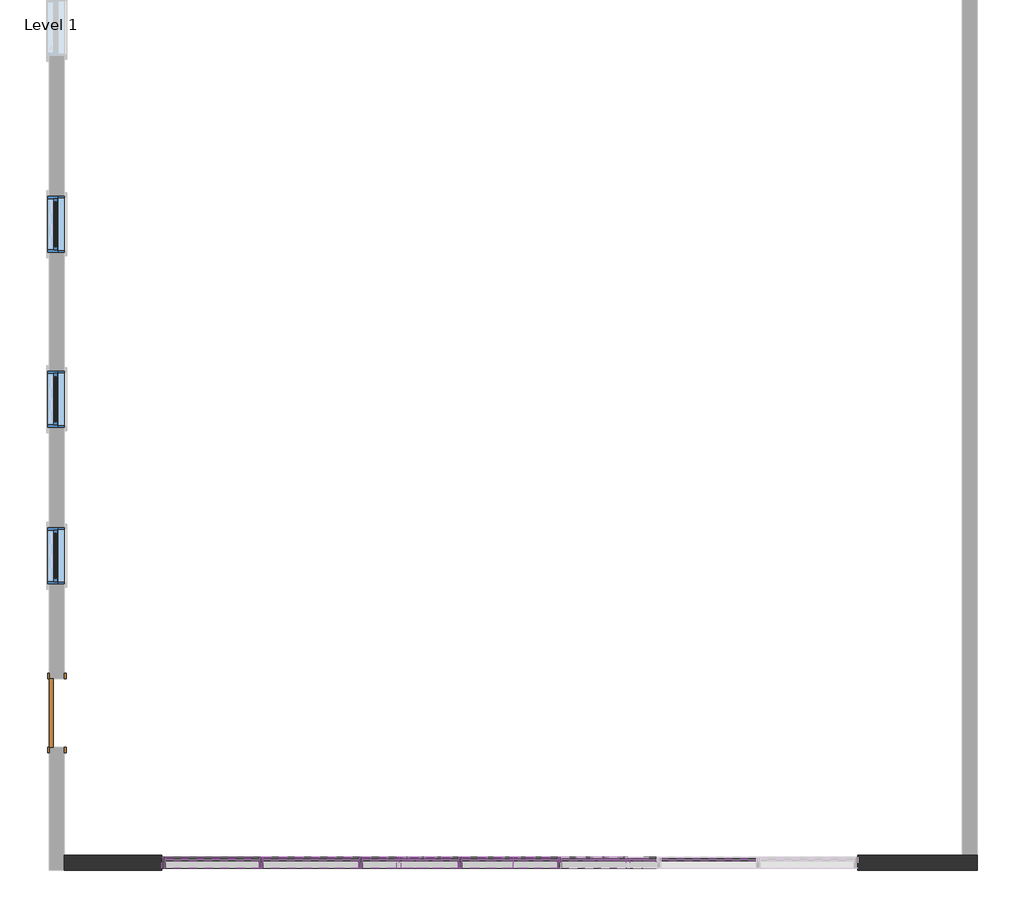
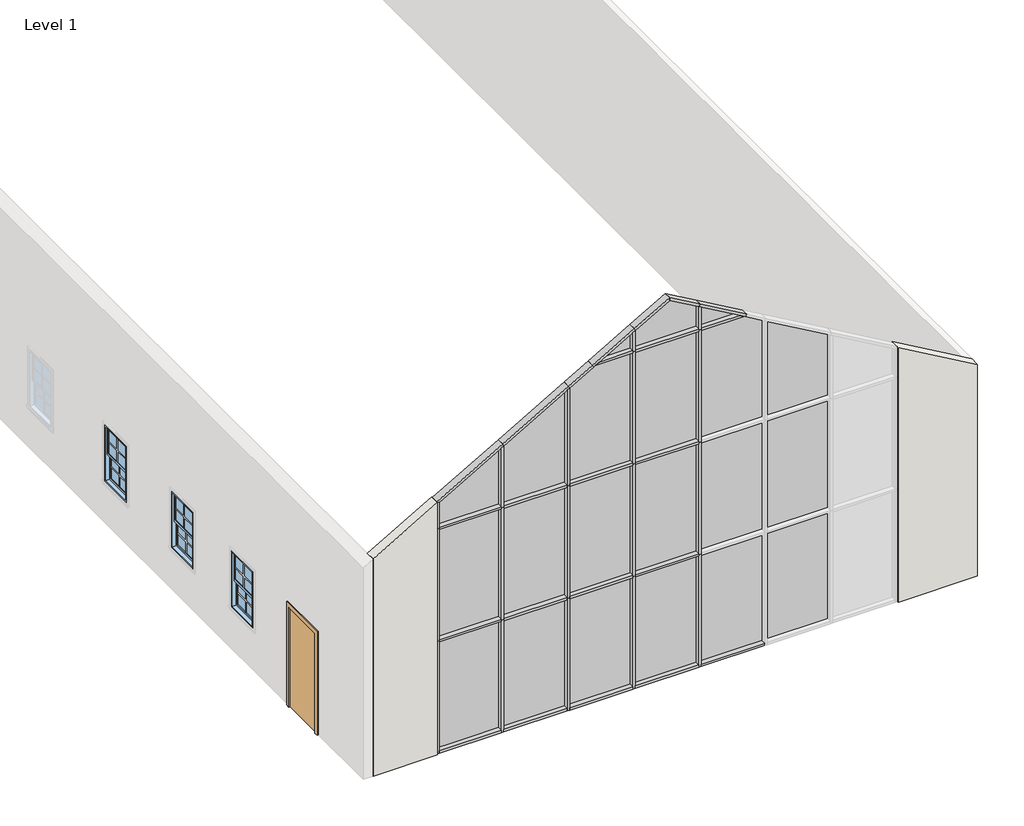
# One storey, part 1 of 2: 40 members, 21 plates, 3 windows, 1 door, 1 wall.
# Revit data of these elements (continued)
# Element 1 (IfcDoor, "M_Single-Flush : 0915 x 2134mm") (continued)
#   Materials on its faces: "Door - Frame", "Door - Panel"
# Elements 2, 3, 4, 5, 6, 7, 8, 9, 10, 11, 12, 13, 14, 15, 16, 17, 18, 19, 20, 21, 22, 23, 24, 25, 26, 27, 28, 29, 30, 31, 32, 33, 34, 35, 36, 37, 38, 39, 40, 41 (IfcMember, "Rectangular Mullion : 50mm x 150mm")
#   Phase Created = New Construction
#   Materials on its faces: "Aluminum"
# Elements 42, 43, 44, 45, 46, 47, 48, 49, 50, 51, 52, 53, 54, 55, 56, 57, 58, 59, 60, 61, 62 (IfcPlate, "System Panel : Glazed")
#   Phase Created = New Construction
#   Materials on its faces: "Glass"
# Element 63 (IfcWall, "Generic - 200mm")
#   Top Offset = 0 mm
#   Base Offset = 0 mm
#   Unconnected Height = 8000 mm
#   wall height = 8000 mm
#   Phase Created = New Construction
#   Base Constraint = Level 1
#   Materials on its faces: "Default Wall"
# Element 64 (IfcWindow, "M_Window-Double-Hung : 750 x 1200mm")
#   Mark = "6"
#   Window Inset = 0 mm
#   Interior Wall Closure = 35.7 mm
#   Frame Extension = 31.75 mm
#   Exterior Wall Closure = 12.7 mm
#   Interior Trim Visibility = yes
#   Indicator Visibility = yes
#   Exterior Trim Visibility = yes
#   Phase Created = New Construction
#   Materials on its faces: "Wood - Stained", "Glass", "Clad - White"
# Element 65 (IfcWindow, "M_Window-Double-Hung : 750 x 1200mm")
#   Mark = "7"
#   Window Inset = 0 mm
#   Interior Wall Closure = 35.7 mm
#   Frame Extension = 31.75 mm
#   Exterior Wall Closure = 12.7 mm
#   Interior Trim Visibility = yes
#   Indicator Visibility = yes
#   Exterior Trim Visibility = yes
#   Phase Created = New Construction
#   Materials on its faces: "Wood - Stained", "Glass", "Clad - White"
# Element 66 (IfcWindow, "M_Window-Double-Hung : 750 x 1200mm")
#   Mark = "8"
#   Window Inset = 0 mm
#   Interior Wall Closure = 35.7 mm
#   Frame Extension = 31.75 mm
#   Exterior Wall Closure = 12.7 mm
#   Interior Trim Visibility = yes
#   Indicator Visibility = yes
#   Exterior Trim Visibility = yes
#   Phase Created = New Construction
#   Materials on its faces: "Wood - Stained", "Glass", "Clad - White"
# Materials
#   "Door - Panel": class "Wood", colour RGB 210 159 95, transparency 0, Cost = 0
#   "Door - Frame": class "Miscellaneous", colour RGB 118 70 51, transparency 0, Cost = 0
#   "Wood - Stained": class "Wood", colour RGB 227 170 128, transparency 0, Cost = 0
#   "Clad - White": class "Wood", colour RGB 242 242 238, transparency 0, Cost = 0
#   "Glass": class "Glass", colour RGB 0 128 192, transparency 0.75, Description = "Soda Lime Glass", Cost = 0
#   "Aluminum": class "Metal", colour RGB 247 247 247, transparency 0, Description = "Aluminum 6061", Cost = 0
#   "Default Wall": class "Miscellaneous", colour RGB 128 128 128, transparency 0, Cost = 0
